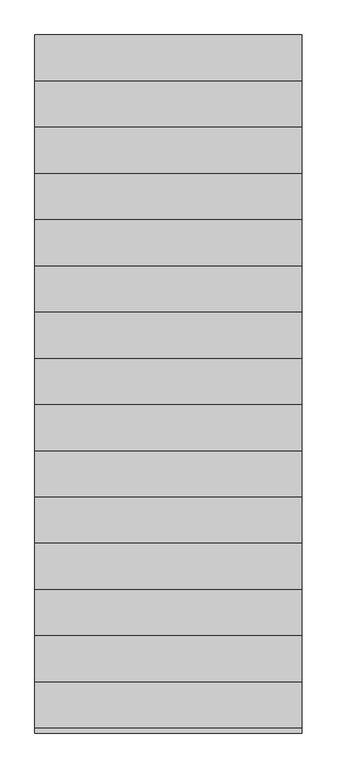
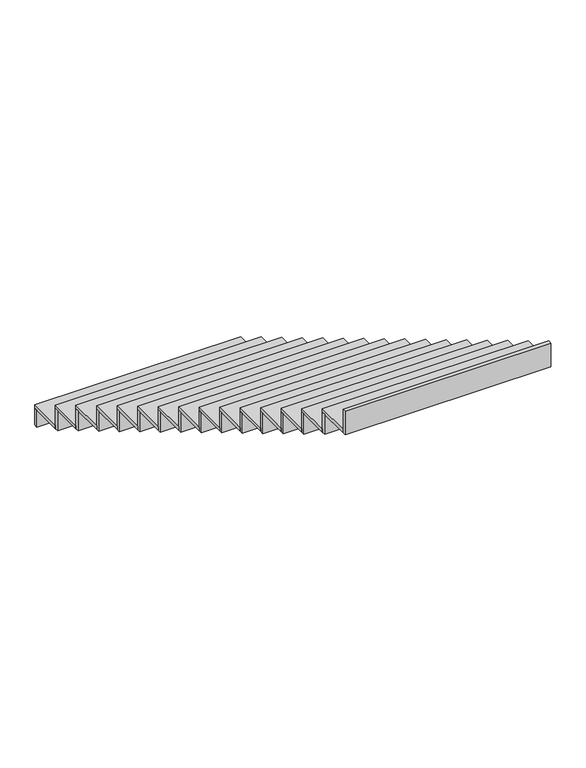
"""IFC4 building model written with IfcOpenShell, lengths in millimetres: stair flight geometry."""

import ifcopenshell
import ifcopenshell.guid

model = None  # the IFC model being written
_history = None  # IfcOwnerHistory: only IFC2X3 demands one
_inside = {}  # id of a spatial element -> (the spatial element, [elements in it])
_under = {}  # id of a project, library or spatial element -> (it, [spatial elements below it])
_declared = {}  # id of a project -> (the project, [libraries it declares])
_typed = {}  # id of a type object -> (the type object, [elements of that type])
_made_of = {}  # id of a material, layer set ... -> (it, [elements and type objects made of it])


def new_model(schema):
    """Start an empty IFC model of exactly this schema.

    Asked for "IFC4X3", IfcOpenShell would pick the latest addendum, in which some entities
    have other attributes; the version numbers below select the first issue.
    IFC2X3 requires an IfcOwnerHistory on every rooted entity: one is made here for all.
    """
    global model, _history
    if schema == "IFC4X3":
        model = ifcopenshell.file(schema_version=(4, 3, 0, 0))
    else:
        model = ifcopenshell.file(schema=schema)
    _inside.clear()
    _under.clear()
    _declared.clear()
    _typed.clear()
    _made_of.clear()
    _history = None
    if model.schema == "IFC2X3":
        org = make("IfcOrganization", Name="unknown")
        user = make(
            "IfcPersonAndOrganization",
            ThePerson=make("IfcPerson", FamilyName="unknown"),
            TheOrganization=org,
        )
        app = make(
            "IfcApplication",
            ApplicationDeveloper=org,
            Version="unknown",
            ApplicationFullName="unknown",
            ApplicationIdentifier="unknown",
        )
        _history = make(
            "IfcOwnerHistory",
            OwningUser=user,
            OwningApplication=app,
            ChangeAction="ADDED",
            CreationDate=0,
        )
    return model


def make(cls, **values):
    """One entity of the class cls with the attributes given. An attribute that is None is left unset."""
    return model.create_entity(
        cls, **{name: value for name, value in values.items() if value is not None}
    )


def rooted(cls, **values):
    """An entity with a GlobalId (a new one), such as an element, a storey or a relation."""
    return make(cls, GlobalId=ifcopenshell.guid.new(), OwnerHistory=_history, **values)


def si_unit(unit_type, name, prefix=None):
    """IfcSIUnit, for example si_unit("LENGTHUNIT", "METRE", prefix="MILLI")."""
    return make("IfcSIUnit", UnitType=unit_type, Prefix=prefix, Name=name)


def assignment(units):
    """IfcUnitAssignment: the units of a project."""
    return None if units is None else make("IfcUnitAssignment", Units=units)


def point(xyz):
    """IfcCartesianPoint."""
    return None if xyz is None else make("IfcCartesianPoint", Coordinates=xyz)


def direction(xyz):
    """IfcDirection."""
    return None if xyz is None else make("IfcDirection", DirectionRatios=xyz)


def frame(location, z_axis=None, x_axis=None):
    """IfcAxis2Placement3D, a coordinate frame: its origin and axes. An axis left out is left unset."""
    return make(
        "IfcAxis2Placement3D",
        Location=point(location),
        Axis=direction(z_axis),
        RefDirection=direction(x_axis),
    )


def origin():
    """The frame at (0, 0, 0) with its axes left unset."""
    return frame((0.0, 0.0, 0.0))


def place(relative_to, where):
    """IfcLocalPlacement: puts the frame where relative to a parent placement (None: the world)."""
    return make(
        "IfcLocalPlacement", PlacementRelTo=relative_to, RelativePlacement=where
    )


def context(
    kind, dimensions, precision=None, world=None, true_north=None, identifier=None
):
    """IfcGeometricRepresentationContext, for example the 3D "Model" context."""
    return make(
        "IfcGeometricRepresentationContext",
        ContextIdentifier=identifier,
        ContextType=kind,
        CoordinateSpaceDimension=dimensions,
        Precision=precision,
        WorldCoordinateSystem=world,
        TrueNorth=true_north,
    )


def project(units=None, contexts=None):
    """IfcProject with its units and contexts."""
    return rooted(
        "IfcProject",
        Name="project",
        RepresentationContexts=contexts,
        UnitsInContext=assignment(units),
    )


def spatial(cls, under=None, at=None, **own):
    """A site, building, storey or space (cls), placed at a placement, below another one or the project."""
    s = rooted(cls, ObjectPlacement=at, **own)
    if under is not None:
        _under.setdefault(under.id(), (under, []))[1].append(s)
    return s


def polyline(points):
    """IfcPolyline through the points."""
    return make("IfcPolyline", Points=[point(p) for p in points])


def outline(outer, holes=None, kind="AREA"):
    """IfcArbitraryClosedProfileDef: a profile drawn as a closed curve; with holes, ...WithVoids."""
    if holes is None:
        return make("IfcArbitraryClosedProfileDef", ProfileType=kind, OuterCurve=outer)
    return make(
        "IfcArbitraryProfileDefWithVoids",
        ProfileType=kind,
        OuterCurve=outer,
        InnerCurves=holes,
    )


def extrude(swept, where, along, depth):
    """IfcExtrudedAreaSolid: the profile swept, set in the frame where, extruded along a direction by depth."""
    return make(
        "IfcExtrudedAreaSolid",
        SweptArea=swept,
        Position=where,
        ExtrudedDirection=direction(along),
        Depth=depth,
    )


def shape(context_of_items, identifier, shape_type, items):
    """IfcShapeRepresentation: the items that make up one representation, for example the "Body"."""
    return make(
        "IfcShapeRepresentation",
        ContextOfItems=context_of_items,
        RepresentationIdentifier=identifier,
        RepresentationType=shape_type,
        Items=items,
    )


def source(mapping_origin, context_of_items, identifier, shape_type, items):
    """IfcRepresentationMap: a shape defined once, which mapped items show again and again."""
    return make(
        "IfcRepresentationMap",
        MappingOrigin=mapping_origin,
        MappedRepresentation=shape(context_of_items, identifier, shape_type, items),
    )


def transform(
    local_origin,
    x_axis=None,
    y_axis=None,
    z_axis=None,
    scale=None,
    scale2=None,
    scale3=None,
    uniform=True,
):
    """IfcCartesianTransformationOperator3D, or its non-uniform kind. x_axis, y_axis, z_axis: its Axis1, 2, 3."""
    if uniform:
        return make(
            "IfcCartesianTransformationOperator3D",
            Axis1=direction(x_axis),
            Axis2=direction(y_axis),
            LocalOrigin=point(local_origin),
            Scale=scale,
            Axis3=direction(z_axis),
        )
    return make(
        "IfcCartesianTransformationOperator3DnonUniform",
        Axis1=direction(x_axis),
        Axis2=direction(y_axis),
        LocalOrigin=point(local_origin),
        Scale=scale,
        Axis3=direction(z_axis),
        Scale2=scale2,
        Scale3=scale3,
    )


def mapped(mapping_source, mapping_target):
    """IfcMappedItem: shows the shape of a source again, moved by a transform."""
    return make(
        "IfcMappedItem", MappingSource=mapping_source, MappingTarget=mapping_target
    )


def made_of(thing, what):
    """Note that an element or type object is made of a material, layer set ...; save() writes the relation."""
    if what is not None:
        _made_of.setdefault(what.id(), (what, []))[1].append(thing)
    return thing


def element(
    cls,
    number,
    at=None,
    inside=None,
    cuts=None,
    type_object=None,
    material=None,
    context=None,
    identifier="Body",
    shape_type=None,
    held_by="IfcProductDefinitionShape",
    body=None,
    shapes=None,
    **own,
):
    """One element of the class cls, such as IfcWall. Its Tag is "e" and its number.

    at: its placement. inside: the storey or other place that contains it. cuts: it is an
    opening in that element (IfcRelVoidsElement). A single representation is given by context,
    identifier, shape_type and body (its items); several are given by shapes. held_by: the class
    of the entity that holds the representations. save() writes the other relations.
    """
    e = rooted(cls, Tag="e%d" % number, ObjectPlacement=at, **own)
    if body is not None:
        shapes = [shape(context, identifier, shape_type, body)]
    if shapes is not None:
        e.Representation = make(held_by, Representations=shapes)
    if inside is not None:
        _inside.setdefault(inside.id(), (inside, []))[1].append(e)
    if cuts is not None:
        rooted(
            "IfcRelVoidsElement", RelatingBuildingElement=cuts, RelatedOpeningElement=e
        )
    if type_object is not None:
        _typed.setdefault(type_object.id(), (type_object, []))[1].append(e)
    return made_of(e, material)


def aggregate(whole, parts):
    """IfcRelAggregates: a whole, such as a stair, and the parts it consists of."""
    return rooted("IfcRelAggregates", RelatingObject=whole, RelatedObjects=parts)


def save(model, path):
    """Write the relations noted so far, then the file.

    IfcRelAggregates (storeys below a building ...), IfcRelContainedInSpatialStructure (elements
    in a storey), IfcRelDefinesByType, IfcRelAssociatesMaterial and IfcRelDeclares: one each for
    every whole, place, type object, material and project.
    """
    for whole, parts in _under.values():
        aggregate(whole, parts)
    for where, things in _inside.values():
        rooted(
            "IfcRelContainedInSpatialStructure",
            RelatedElements=things,
            RelatingStructure=where,
        )
    for kind, things in _typed.values():
        rooted("IfcRelDefinesByType", RelatedObjects=things, RelatingType=kind)
    for what, things in _made_of.values():
        rooted("IfcRelAssociatesMaterial", RelatedObjects=things, RelatingMaterial=what)
    for by, libraries in _declared.values():
        rooted("IfcRelDeclares", RelatingContext=by, RelatedDefinitions=libraries)
    model.write(path)


def stair_flight_12b22758(model_context):
    return source(origin(), model_context, "Body", "SweptSolid", [
        extrude(outline(polyline([(52915.0, -1730.0), (52915.0, -1700.0), (54650.0, -1700.0), (54650.0, -1730.0), (52915.0, -1730.0)])), frame((0.0, 0.0, 7730.0), z_axis=(0.0, 0.0, 1.0), x_axis=(1.0, 0.0, 0.0)), (0.0, 0.0, 1.0), 149.375),
        extrude(outline(polyline([(54650.0, -2000.0), (52915.0, -2000.0), (52915.0, -1700.0), (54650.0, -1700.0), (54650.0, -2000.0)])), frame((0.0, 0.0, 7879.375), z_axis=(0.0, 0.0, 1.0), x_axis=(1.0, 0.0, 0.0)), (0.0, 0.0, 1.0), 30.0),
        extrude(outline(polyline([(52915.0, -2030.0), (52915.0, -2000.0), (54650.0, -2000.0), (54650.0, -2030.0), (52915.0, -2030.0)])), frame((0.0, 0.0, 7879.375), z_axis=(0.0, 0.0, 1.0), x_axis=(1.0, 0.0, 0.0)), (0.0, 0.0, 1.0), 179.375),
        extrude(outline(polyline([(54650.0, -2300.0), (52915.0, -2300.0), (52915.0, -2000.0), (54650.0, -2000.0), (54650.0, -2300.0)])), frame((0.0, 0.0, 8058.75), z_axis=(0.0, 0.0, 1.0), x_axis=(1.0, 0.0, 0.0)), (0.0, 0.0, 1.0), 30.0),
        extrude(outline(polyline([(52915.0, -2330.0), (52915.0, -2300.0), (54650.0, -2300.0), (54650.0, -2330.0), (52915.0, -2330.0)])), frame((0.0, 0.0, 8058.75), z_axis=(0.0, 0.0, 1.0), x_axis=(1.0, 0.0, 0.0)), (0.0, 0.0, 1.0), 179.375),
        extrude(outline(polyline([(54650.0, -2600.0), (52915.0, -2600.0), (52915.0, -2300.0), (54650.0, -2300.0), (54650.0, -2600.0)])), frame((0.0, 0.0, 8238.125), z_axis=(0.0, 0.0, 1.0), x_axis=(1.0, 0.0, 0.0)), (0.0, 0.0, 1.0), 30.0),
        extrude(outline(polyline([(52915.0, -2630.0), (52915.0, -2600.0), (54650.0, -2600.0), (54650.0, -2630.0), (52915.0, -2630.0)])), frame((0.0, 0.0, 8238.125), z_axis=(0.0, 0.0, 1.0), x_axis=(1.0, 0.0, 0.0)), (0.0, 0.0, 1.0), 179.375),
        extrude(outline(polyline([(54650.0, -2900.0), (52915.0, -2900.0), (52915.0, -2600.0), (54650.0, -2600.0), (54650.0, -2900.0)])), frame((0.0, 0.0, 8417.5), z_axis=(0.0, 0.0, 1.0), x_axis=(1.0, 0.0, 0.0)), (0.0, 0.0, 1.0), 30.0),
        extrude(outline(polyline([(52915.0, -2930.0), (52915.0, -2900.0), (54650.0, -2900.0), (54650.0, -2930.0), (52915.0, -2930.0)])), frame((0.0, 0.0, 8417.5), z_axis=(0.0, 0.0, 1.0), x_axis=(1.0, 0.0, 0.0)), (0.0, 0.0, 1.0), 179.375),
        extrude(outline(polyline([(54650.0, -3200.0), (52915.0, -3200.0), (52915.0, -2900.0), (54650.0, -2900.0), (54650.0, -3200.0)])), frame((0.0, 0.0, 8596.875), z_axis=(0.0, 0.0, 1.0), x_axis=(1.0, 0.0, 0.0)), (0.0, 0.0, 1.0), 30.0),
        extrude(outline(polyline([(52915.0, -3230.0), (52915.0, -3200.0), (54650.0, -3200.0), (54650.0, -3230.0), (52915.0, -3230.0)])), frame((0.0, 0.0, 8596.875), z_axis=(0.0, 0.0, 1.0), x_axis=(1.0, 0.0, 0.0)), (0.0, 0.0, 1.0), 179.375),
        extrude(outline(polyline([(54650.0, -3500.0), (52915.0, -3500.0), (52915.0, -3200.0), (54650.0, -3200.0), (54650.0, -3500.0)])), frame((0.0, 0.0, 8776.25), z_axis=(0.0, 0.0, 1.0), x_axis=(1.0, 0.0, 0.0)), (0.0, 0.0, 1.0), 30.0),
        extrude(outline(polyline([(52915.0, -3530.0), (52915.0, -3500.0), (54650.0, -3500.0), (54650.0, -3530.0), (52915.0, -3530.0)])), frame((0.0, 0.0, 8776.25), z_axis=(0.0, 0.0, 1.0), x_axis=(1.0, 0.0, 0.0)), (0.0, 0.0, 1.0), 179.375),
        extrude(outline(polyline([(54650.0, -3800.0), (52915.0, -3800.0), (52915.0, -3500.0), (54650.0, -3500.0), (54650.0, -3800.0)])), frame((0.0, 0.0, 8955.625), z_axis=(0.0, 0.0, 1.0), x_axis=(1.0, 0.0, 0.0)), (0.0, 0.0, 1.0), 30.0),
        extrude(outline(polyline([(52915.0, -3830.0), (52915.0, -3800.0), (54650.0, -3800.0), (54650.0, -3830.0), (52915.0, -3830.0)])), frame((0.0, 0.0, 8955.625), z_axis=(0.0, 0.0, 1.0), x_axis=(1.0, 0.0, 0.0)), (0.0, 0.0, 1.0), 179.375),
        extrude(outline(polyline([(54650.0, -4100.0), (52915.0, -4100.0), (52915.0, -3800.0), (54650.0, -3800.0), (54650.0, -4100.0)])), frame((0.0, 0.0, 9135.0), z_axis=(0.0, 0.0, 1.0), x_axis=(1.0, 0.0, 0.0)), (0.0, 0.0, 1.0), 30.0),
        extrude(outline(polyline([(52915.0, -4130.0), (52915.0, -4100.0), (54650.0, -4100.0), (54650.0, -4130.0), (52915.0, -4130.0)])), frame((0.0, 0.0, 9135.0), z_axis=(0.0, 0.0, 1.0), x_axis=(1.0, 0.0, 0.0)), (0.0, 0.0, 1.0), 179.375),
        extrude(outline(polyline([(54650.0, -4400.0), (52915.0, -4400.0), (52915.0, -4100.0), (54650.0, -4100.0), (54650.0, -4400.0)])), frame((0.0, 0.0, 9314.375), z_axis=(0.0, 0.0, 1.0), x_axis=(1.0, 0.0, 0.0)), (0.0, 0.0, 1.0), 30.0),
        extrude(outline(polyline([(52915.0, -4430.0), (52915.0, -4400.0), (54650.0, -4400.0), (54650.0, -4430.0), (52915.0, -4430.0)])), frame((0.0, 0.0, 9314.375), z_axis=(0.0, 0.0, 1.0), x_axis=(1.0, 0.0, 0.0)), (0.0, 0.0, 1.0), 179.375),
        extrude(outline(polyline([(54650.0, -4700.0), (52915.0, -4700.0), (52915.0, -4400.0), (54650.0, -4400.0), (54650.0, -4700.0)])), frame((0.0, 0.0, 9493.75), z_axis=(0.0, 0.0, 1.0), x_axis=(1.0, 0.0, 0.0)), (0.0, 0.0, 1.0), 30.0),
        extrude(outline(polyline([(52915.0, -4730.0), (52915.0, -4700.0), (54650.0, -4700.0), (54650.0, -4730.0), (52915.0, -4730.0)])), frame((0.0, 0.0, 9493.75), z_axis=(0.0, 0.0, 1.0), x_axis=(1.0, 0.0, 0.0)), (0.0, 0.0, 1.0), 179.375),
        extrude(outline(polyline([(54650.0, -5000.0), (52915.0, -5000.0), (52915.0, -4700.0), (54650.0, -4700.0), (54650.0, -5000.0)])), frame((0.0, 0.0, 9673.125), z_axis=(0.0, 0.0, 1.0), x_axis=(1.0, 0.0, 0.0)), (0.0, 0.0, 1.0), 30.0),
        extrude(outline(polyline([(52915.0, -5030.0), (52915.0, -5000.0), (54650.0, -5000.0), (54650.0, -5030.0), (52915.0, -5030.0)])), frame((0.0, 0.0, 9673.125), z_axis=(0.0, 0.0, 1.0), x_axis=(1.0, 0.0, 0.0)), (0.0, 0.0, 1.0), 179.375),
        extrude(outline(polyline([(54650.0, -5300.0), (52915.0, -5300.0), (52915.0, -5000.0), (54650.0, -5000.0), (54650.0, -5300.0)])), frame((0.0, 0.0, 9852.5), z_axis=(0.0, 0.0, 1.0), x_axis=(1.0, 0.0, 0.0)), (0.0, 0.0, 1.0), 30.0),
        extrude(outline(polyline([(52915.0, -5330.0), (52915.0, -5300.0), (54650.0, -5300.0), (54650.0, -5330.0), (52915.0, -5330.0)])), frame((0.0, 0.0, 9852.5), z_axis=(0.0, 0.0, 1.0), x_axis=(1.0, 0.0, 0.0)), (0.0, 0.0, 1.0), 179.375),
        extrude(outline(polyline([(54650.0, -5600.0), (52915.0, -5600.0), (52915.0, -5300.0), (54650.0, -5300.0), (54650.0, -5600.0)])), frame((0.0, 0.0, 10031.875), z_axis=(0.0, 0.0, 1.0), x_axis=(1.0, 0.0, 0.0)), (0.0, 0.0, 1.0), 30.0),
        extrude(outline(polyline([(52915.0, -5630.0), (52915.0, -5600.0), (54650.0, -5600.0), (54650.0, -5630.0), (52915.0, -5630.0)])), frame((0.0, 0.0, 10031.875), z_axis=(0.0, 0.0, 1.0), x_axis=(1.0, 0.0, 0.0)), (0.0, 0.0, 1.0), 179.375),
        extrude(outline(polyline([(54650.0, -5900.0), (52915.0, -5900.0), (52915.0, -5600.0), (54650.0, -5600.0), (54650.0, -5900.0)])), frame((0.0, 0.0, 10211.25), z_axis=(0.0, 0.0, 1.0), x_axis=(1.0, 0.0, 0.0)), (0.0, 0.0, 1.0), 30.0),
        extrude(outline(polyline([(52915.0, -5930.0), (52915.0, -5900.0), (54650.0, -5900.0), (54650.0, -5930.0), (52915.0, -5930.0)])), frame((0.0, 0.0, 10211.25), z_axis=(0.0, 0.0, 1.0), x_axis=(1.0, 0.0, 0.0)), (0.0, 0.0, 1.0), 179.375),
        extrude(outline(polyline([(52915.0, -6230.0), (52915.0, -6200.0), (54650.0, -6200.0), (54650.0, -6230.0), (52915.0, -6230.0)])), frame((0.0, 0.0, 10390.625), z_axis=(0.0, 0.0, 1.0), x_axis=(1.0, 0.0, 0.0)), (0.0, 0.0, 1.0), 209.375),
        extrude(outline(polyline([(54650.0, -6200.0), (52915.0, -6200.0), (52915.0, -5900.0), (54650.0, -5900.0), (54650.0, -6200.0)])), frame((0.0, 0.0, 10390.625), z_axis=(0.0, 0.0, 1.0), x_axis=(1.0, 0.0, 0.0)), (0.0, 0.0, 1.0), 30.0),
    ])


if __name__ == "__main__":
    model = new_model("IFC4")
    model_context = context("Model", 3, world=origin())
    ifc_project = project(units=[si_unit("LENGTHUNIT", "METRE", prefix="MILLI")], contexts=[model_context])
    site = spatial("IfcSite", under=ifc_project)
    building = spatial("IfcBuilding", under=site)
    placement = place(None, origin())
    stair_flight_shape = stair_flight_12b22758(model_context)
    element("IfcStairFlight", 1, at=placement, inside=building, context=model_context, shape_type="MappedRepresentation", body=[
        mapped(stair_flight_shape, transform((0.0, 0.0, 0.0), x_axis=(1.0, 0.0, 0.0), y_axis=(0.0, 1.0, 0.0), z_axis=(0.0, 0.0, 1.0))),
    ])
    save(model, "model.ifc")

# Revit data of these elements
# Element 1 (IfcStairFlight)
#   Materials on its faces: "00_Finish_Deco Tile"
# Materials
#   "00_Finish_Deco Tile": class "Finish", colour RGB 245 245 245, transparency 0, Description = "Ceramic Tile", Cost = 0
